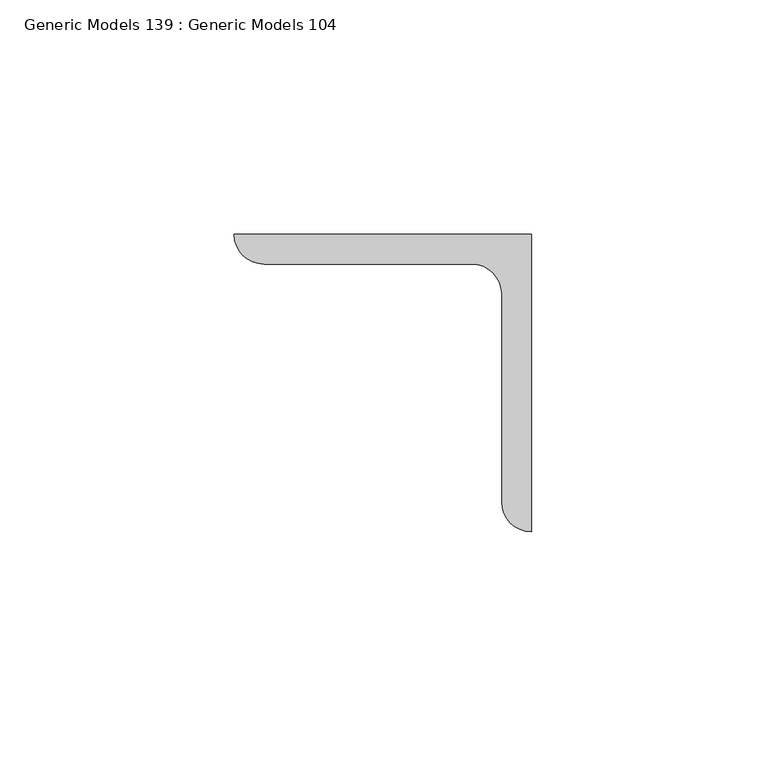
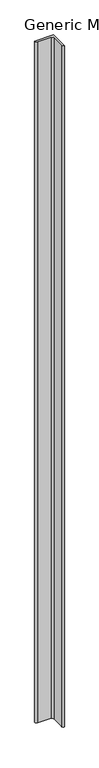
"""IFC4 building model written with IfcOpenShell, lengths in millimetres: proxy geometry, Generic Models 139 : Generic Models 104."""

from ifc_helpers import new_model, si_unit, point, frame, frame_2d, origin, place, context, project, spatial, polyline, circle_curve, trimmed, segment, composite_curve, outline, extrude, source, transform, mapped, element, save


def generic_models_139_generic_models_104_cae5c93c(model_context):
    return source(origin(), model_context, "Body", "SweptSolid", [
        extrude(outline(composite_curve([segment(polyline([(31276.6040778, 41071.1196612), (31276.6040778, 41007.6196612)]), True, "CONTINUOUS"), segment(trimmed(circle_curve(frame_2d((31276.6040778, 41013.9696612)), 6.35), [point((31276.6040778, 41007.6196612))], [point((31270.2540778, 41013.9696612))], False, "CARTESIAN"), True, "CONTINUOUS"), segment(polyline([(31270.2540778, 41013.9696612), (31270.2540778, 41058.4196612)]), True, "CONTINUOUS"), segment(trimmed(circle_curve(frame_2d((31263.9040778, 41058.4196612)), 6.35), [point((31270.2540778, 41058.4196612))], [point((31263.9040778, 41064.7696612))], True, "CARTESIAN"), True, "CONTINUOUS"), segment(polyline([(31263.9040778, 41064.7696612), (31219.4540778, 41064.7696612)]), True, "CONTINUOUS"), segment(trimmed(circle_curve(frame_2d((31219.4540778, 41071.1196612)), 6.35), [point((31219.4540778, 41064.7696612))], [point((31213.1040778, 41071.1196612))], False, "CARTESIAN"), True, "CONTINUOUS"), segment(polyline([(31213.1040778, 41071.1196612), (31276.6040778, 41071.1196612)]), True, "CONTINUOUS")], self_intersect=False)), frame((0.0, 0.0, 266407.9), z_axis=(0.0, 0.0, 1.0), x_axis=(1.0, 0.0, 0.0)), (0.0, 0.0, 1.0), 2432.1044757),
    ])


if __name__ == "__main__":
    model = new_model("IFC4")
    model_context = context("Model", 3, world=origin())
    ifc_project = project(units=[si_unit("LENGTHUNIT", "METRE", prefix="MILLI")], contexts=[model_context])
    site = spatial("IfcSite", under=ifc_project)
    building = spatial("IfcBuilding", under=site)
    placement = place(None, origin())
    generic_models_139_generic_models_104_shape = generic_models_139_generic_models_104_cae5c93c(model_context)
    element("IfcBuildingElementProxy", 1, Name="Generic Models 139 : Generic Models 104", ObjectType="Generic Models 139 : Generic Models 104", at=placement, inside=building, context=model_context, shape_type="MappedRepresentation", body=[
        mapped(generic_models_139_generic_models_104_shape, transform((0.0, 0.0, 0.0), x_axis=(1.0, 0.0, 0.0), y_axis=(0.0, 1.0, 0.0), z_axis=(0.0, 0.0, 1.0))),
    ])
    save(model, "model.ifc")

# Revit data of these elements
# Element 1 (IfcBuildingElementProxy, "Generic Models 139 : Generic Models 104")
#   Materials on its faces: "(2) BACK/BACK GALVANIZED ANGLES (2) L2 1/2 X 2 1/2 X 1/4\")"
# Materials
#   "(2) BACK/BACK GALVANIZED ANGLES (2) L2 1/2 X 2 1/2 X 1/4\")": class "Unassigned", colour RGB 211 211 211, transparency 0, Cost = 0
